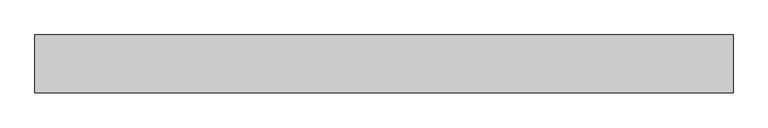
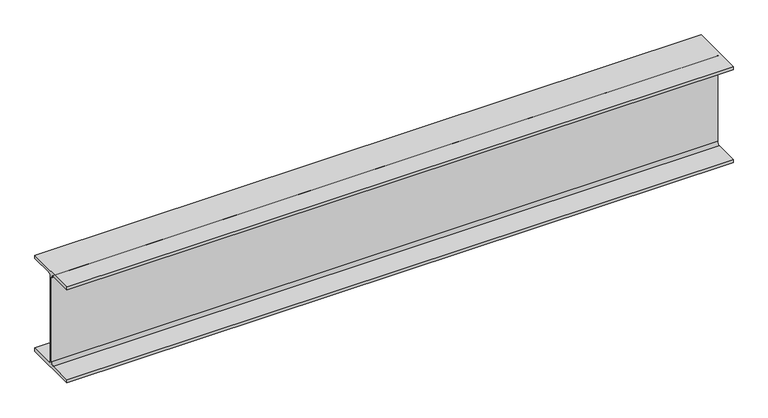
"""IFC4 building model written with IfcOpenShell, lengths in millimetres: beam geometry, Old_Steel Beam_H-KSD3502 : H_SB_ASB_H-194×150x6x9."""

from ifc_helpers import new_model, si_unit, point, frame, frame_2d, origin, place, context, project, spatial, polyline, circle_curve, trimmed, segment, composite_curve, outline, extrude, source, transform, mapped, element, save


def beam_df7a2f66(model_context):
    return source(origin(), model_context, "Body", "SweptSolid", [
        extrude(outline(composite_curve([segment(polyline([(82.5, -141.5), (82.5, -151.7), (-82.5, -151.7), (-82.5, -141.5), (-11.9, -141.5)]), True, "CONTINUOUS"), segment(trimmed(circle_curve(frame_2d((-11.9, -132.6)), 8.9), [point((-11.9, -141.5))], [point((-3.0, -132.6))], True, "CARTESIAN"), True, "CONTINUOUS"), segment(polyline([(-3.0, -132.6), (-3.0, 132.6)]), True, "CONTINUOUS"), segment(trimmed(circle_curve(frame_2d((-11.9, 132.6)), 8.9), [point((-3.0, 132.6))], [point((-11.9, 141.5))], True, "CARTESIAN"), True, "CONTINUOUS"), segment(polyline([(-11.9, 141.5), (-82.5, 141.5), (-82.5, 151.7), (82.5, 151.7), (82.5, 141.5), (11.9, 141.5)]), True, "CONTINUOUS"), segment(trimmed(circle_curve(frame_2d((11.9, 132.6)), 8.9), [point((11.9, 141.5))], [point((3.0, 132.6))], True, "CARTESIAN"), True, "CONTINUOUS"), segment(polyline([(3.0, 132.6), (3.0, -132.6)]), True, "CONTINUOUS"), segment(trimmed(circle_curve(frame_2d((11.9, -132.6)), 8.9), [point((3.0, -132.6))], [point((11.9, -141.5))], True, "CARTESIAN"), True, "CONTINUOUS"), segment(polyline([(11.9, -141.5), (82.5, -141.5)]), True, "CONTINUOUS")], self_intersect=False)), frame((-1120.7772651, 0.0, 0.0), z_axis=(1.0, 0.0, 0.0), x_axis=(0.0, 1.0, 0.0)), (0.0, 0.0, 1.0), 1987.9940387),
    ])


if __name__ == "__main__":
    model = new_model("IFC4")
    model_context = context("Model", 3, world=origin())
    ifc_project = project(units=[si_unit("LENGTHUNIT", "METRE", prefix="MILLI")], contexts=[model_context])
    site = spatial("IfcSite", under=ifc_project)
    building = spatial("IfcBuilding", under=site)
    placement = place(None, origin())
    beam_shape = beam_df7a2f66(model_context)
    element("IfcBeam", 1, ObjectType="Old_Steel Beam_H-KSD3502 : H_SB_ASB_H-194×150x6x9", at=placement, inside=building, context=model_context, shape_type="MappedRepresentation", body=[
        mapped(beam_shape, transform((0.0, 0.0, 0.0), x_axis=(1.0, 0.0, 0.0), y_axis=(0.0, 1.0, 0.0), z_axis=(0.0, 0.0, 1.0))),
    ])
    save(model, "model.ifc")

# Revit data of these elements
# Type "Old_Steel Beam_H-KSD3502 : H_SB_ASB_H-194×150x6x9"
#   Width = 15.0 cm
#   Web Thickness = 0.6 cm
#   Web Fillet = 1.3 cm
#   Warping Constant = 43316.0 cm⁶
#   Torsional Moment of Inertia = 8.622 cm⁴
#   Torsional Modulus = 1.0 cm³
#   Section Area = 39.01 cm²
#   Plastic Modulus weak axis = 104.0 cm³
#   Plastic Modulus strong axis = 309.0 cm³
#   Perimeter = 0.95 m²/m
#   Nominal Weight = 30.60 kgf/m
#   Moment of Inertia weak axis = 507.00 cm⁴
#   Moment of Inertia strong axis = 2690.00 cm⁴
#   Height = 19.4 cm
#   Flange Thickness = 0.9 cm
#   Elastic Modulus weak axis = 67.6 cm³
#   Elastic Modulus strong axis = 277.0 cm³
#   Centroid Vertical = 9.7 cm
#   Centroid Horizontal = 7.5 cm
#   Length [instance default] = 1.5240 m
#   Structural Material [instance default] = Steel, 45-345
#   Assembly Code = ""
# Element 1 (IfcBeam, "Old_Steel Beam_H-KSD3502 : H_SB_ASB_H-194×150x6x9")
#   Structural Material = none
# Materials
#   "Steel, 45-345": class "Metal", colour RGB 189 187 185, transparency 0, Description = "Steel 345 MPa", Cost = 0
